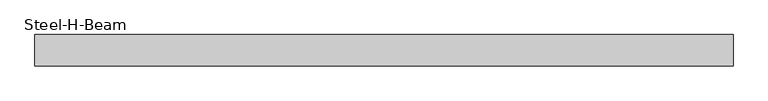
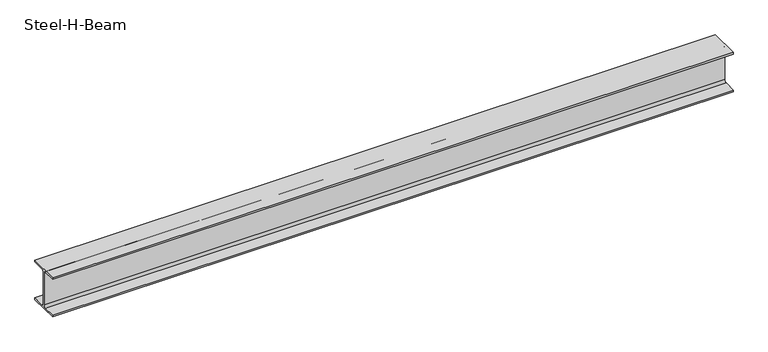
"""IFC4 building model written with IfcOpenShell, lengths in millimetres: beam geometry, Steel-H-Beam : BM121_H-340×250x9x14."""

from ifc_helpers import new_model, si_unit, point, frame, frame_2d, origin, place, context, project, spatial, polyline, circle_curve, trimmed, segment, composite_curve, outline, extrude, source, transform, mapped, element, save


def steel_h_beam_3a09662f(model_context):
    return source(origin(), model_context, "Body", "SweptSolid", [
        extrude(outline(composite_curve([segment(polyline([(125.0, -156.0), (125.0, -170.0), (-125.0, -170.0), (-125.0, -156.0), (-24.5, -156.0)]), True, "CONTINUOUS"), segment(trimmed(circle_curve(frame_2d((-24.5, -136.0)), 20.0), [point((-24.5, -156.0))], [point((-4.5, -136.0))], True, "CARTESIAN"), True, "CONTINUOUS"), segment(polyline([(-4.5, -136.0), (-4.5, 136.0)]), True, "CONTINUOUS"), segment(trimmed(circle_curve(frame_2d((-24.5, 136.0)), 20.0), [point((-4.5, 136.0))], [point((-24.5, 156.0))], True, "CARTESIAN"), True, "CONTINUOUS"), segment(polyline([(-24.5, 156.0), (-125.0, 156.0), (-125.0, 170.0), (125.0, 170.0), (125.0, 156.0), (24.5, 156.0)]), True, "CONTINUOUS"), segment(trimmed(circle_curve(frame_2d((24.5, 136.0)), 20.0), [point((24.5, 156.0))], [point((4.5, 136.0))], True, "CARTESIAN"), True, "CONTINUOUS"), segment(polyline([(4.5, 136.0), (4.5, -136.0)]), True, "CONTINUOUS"), segment(trimmed(circle_curve(frame_2d((24.5, -136.0)), 20.0), [point((4.5, -136.0))], [point((24.5, -156.0))], True, "CARTESIAN"), True, "CONTINUOUS"), segment(polyline([(24.5, -156.0), (125.0, -156.0)]), True, "CONTINUOUS")], self_intersect=False)), frame((-2768.817822, 0.0, 0.0), z_axis=(1.0, 0.0, 0.0), x_axis=(0.0, 1.0, 0.0)), (0.0, 0.0, 1.0), 5580.2433846),
    ])


if __name__ == "__main__":
    model = new_model("IFC4")
    model_context = context("Model", 3, world=origin())
    ifc_project = project(units=[si_unit("LENGTHUNIT", "METRE", prefix="MILLI")], contexts=[model_context])
    site = spatial("IfcSite", under=ifc_project)
    building = spatial("IfcBuilding", under=site)
    placement = place(None, origin())
    steel_h_beam_shape = steel_h_beam_3a09662f(model_context)
    element("IfcBeam", 1, ObjectType="Steel-H-Beam : BM121_H-340×250x9x14", at=placement, inside=building, context=model_context, shape_type="MappedRepresentation", body=[
        mapped(steel_h_beam_shape, transform((0.0, 0.0, 0.0), x_axis=(1.0, 0.0, 0.0), y_axis=(0.0, 1.0, 0.0), z_axis=(0.0, 0.0, 1.0))),
    ])
    save(model, "model.ifc")

# Revit data of these elements
# Type "Steel-H-Beam : BM121_H-340×250x9x14"
#   Surface Area = 1.62766 m²/m
#   Section Area = 101.514 cm²
#   Mass per Unit Length = 79.6882 kg/m
#   Length [instance default] = 3000 mm
#   B = 250 mm
#   H = 340 mm
#   r = 20 mm
#   tw = 9 mm
#   tf = 14 mm
#   hec_material4 [instance default] = none
#   hec_material3 [instance default] = none
#   hec_material2 [instance default] = none
#   hec_material1 [instance default] = none
#   Structural Material [instance default] = Steel, 45-345
#   Assembly Code = ""
# Element 1 (IfcBeam, "Steel-H-Beam : BM121_H-340×250x9x14")
#   hec_material4 = S01AA010-00002_Main Steel Structure Fabrication Work_Shelter/Building_Steel Painting/Coating_for Fireproofed Steel Surface, Surface Preparation & Primer Coat
#   hec_material3 = F01AC000-00002_Building/Shelter Fire Proofing Work_Intumescent Coating Type_1 hr. rating (UL 1709))
#   hec_material2 = S01AA010-00002_Main Steel Structure Fabrication Work_Shelter/Building_Steel Painting/Coating_for Fireproofed Steel Surface, Surface Preparation & Primer Coat
#   hec_material1 = S03AA028-00001_Main Steel Structure Erection Work_Shelter/Building_Medium Steel
#   Structural Material = S01AA002-00001_Main Steel Structure Fabrication Work_Shelter/Building_Medium Steel - Standard
#   Materials on its faces: "S01AA002-00001_Main Steel Structure Fabrication Work_Shelter/Building_Medium Steel - Standard"
# Materials
#   "Steel, 45-345": class "Metal", colour RGB 189 187 185, transparency 0, Description = "Steel 345 MPa", Cost = 0
#   "S01AA002-00001_Main Steel Structure Fabrication Work_Shelter/Building_Medium Steel - Standard": class "Metal", colour RGB 120 120 120, transparency 0, Comments = "(90KG/M>Weight≥30KG/M)", Description = "Structural steel 50ksi", W00) Work Master Code = "S01AA002-0001", W01) Work Master_Lv1 = "Main Steel Structure Fabrication Work", W02) Work Master_Lv2 = "Shelter/Building", W03) Work Master_Spec.1 = "Medium Steel - Standard (90KG/M>Weight≥30KG/M)", Cost = 0
#   "S01AA010-00002_Main Steel Structure Fabrication Work_Shelter/Building_Steel Painting/Coating_for Fireproofed Steel Surface, Surface Preparation & Primer Coat": class "Metal", colour RGB 120 120 120, transparency 0, Description = "Paint finished steel", W00) Work Master Code = "SS01AA010-00002", W01) Work Master_Lv1 = "Main Steel Structure Fabrication Work", W02) Work Master_Lv2 = "Shelter/Building", W03) Work Master_Spec.1 = "Steel Painting/Coating", W04) Work Master_Spec.2 = "for Fireproofed Steel Surface, Surface Preparation & Primer Coat", Cost = 0
#   "F01AC000-00002_Building/Shelter Fire Proofing Work_Intumescent Coating Type_1 hr. rating (UL 1709))": class "Metal", colour RGB 255 128 128, transparency 0, Description = "Paint finished steel", W00) Work Master Code = "F01AC000-00002", W01) Work Master_Lv1 = "Building/Shelter Fire Proofing Work", W02) Work Master_Lv2 = "Intumescent Coating Type", W03) Work Master_Spec.1 = "1 hr. rating (UL 1709)", Cost = 0
#   "S03AA028-00001_Main Steel Structure Erection Work_Shelter/Building_Medium Steel": class "Metal", colour RGB 120 120 120, transparency 0, Comments = "(90KG/M>Weight≥30KG/M)", Description = "Structural steel 50ksi", W00) Work Master Code = "S03AA028-0001", W01) Work Master_Lv1 = "Main Steel Structure Erection Work", W02) Work Master_Lv2 = "Shelter/Building", W03) Work Master_Spec.1 = "Medium Steel (90KG/M>Weight≥30KG/M)", Cost = 0
